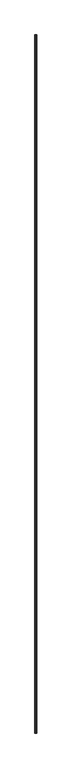
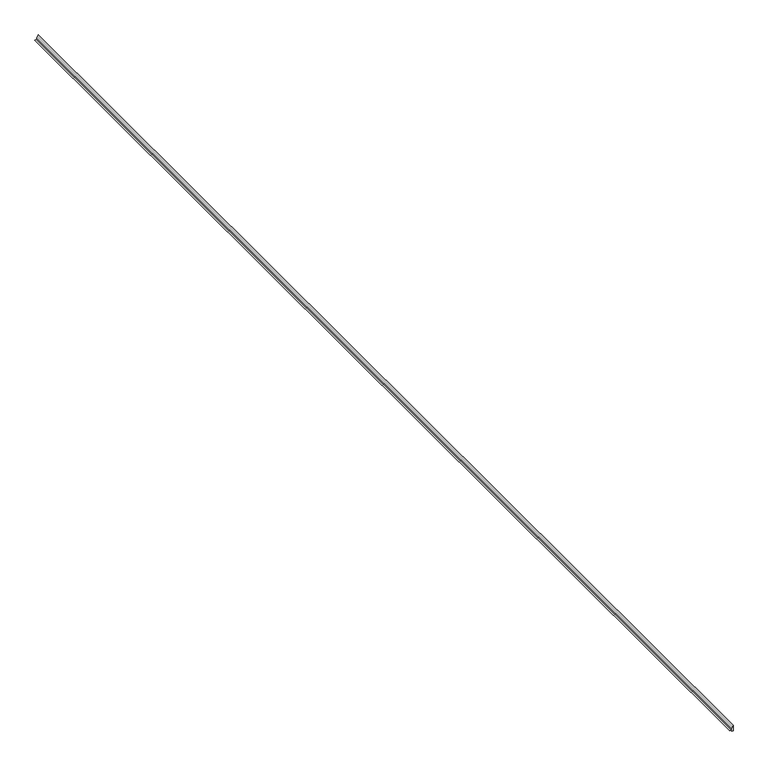
"""IFC4 building model written with IfcOpenShell, lengths in millimetres: proxy geometry, Generic Models 3:Generic Models 2:312240:Generic Models 2:312240 : Generic Models 3:Generic Models 2:312240:7 : Generic Models 3:Generic Models 2:312240:Generic Models 2:312240 : Generic Models 3:Generic Models 2:312240:300533."""

from ifc_helpers import new_model, si_unit, frame, origin, place, context, project, spatial, polyline, outline, extrude, source, transform, mapped, element, save


def generic_models_042a4f2a(model_context):
    return source(origin(), model_context, "Body", "SweptSolid", [
        extrude(outline(polyline([(0.0, 667585.4117239), (-2.5068284, 667585.4117239), (-2.5068284, 667587.6995663), (0.0, 667587.6995663), (9.4480138, 667587.6995663), (2.7766894, 667585.0041763), (1.5875, 667583.8149868), (0.0, 667581.0653562), (0.0, 667585.4117239)])), frame((0.0, -568496.2038841, 0.0), z_axis=(0.0, 1.0, 0.0), x_axis=(0.0, 0.0, 1.0)), (0.0, 0.0, 1.0), 2438.4),
    ])


if __name__ == "__main__":
    model = new_model("IFC4")
    model_context = context("Model", 3, world=origin())
    ifc_project = project(units=[si_unit("LENGTHUNIT", "METRE", prefix="MILLI")], contexts=[model_context])
    site = spatial("IfcSite", under=ifc_project)
    building = spatial("IfcBuilding", under=site)
    placement = place(None, origin())
    generic_models_shape = generic_models_042a4f2a(model_context)
    element("IfcBuildingElementProxy", 1, Name="Generic Models 3:Generic Models 2:312240:Generic Models 2:312240 : Generic Models 3:Generic Models 2:312240:7 : Generic Models 3:Generic Models 2:312240:Generic Models 2:312240 : Generic Models 3:Generic Models 2:312240:300533", ObjectType="Generic Models 3:Generic Models 2:312240:Generic Models 2:312240 : Generic Models 3:Generic Models 2:312240:7 : Generic Models 3:Generic Models 2:312240:Generic Models 2:312240 : Generic Models 3:Generic Models 2:312240:300533", at=placement, inside=building, context=model_context, shape_type="MappedRepresentation", body=[
        mapped(generic_models_shape, transform((0.0, 0.0, 0.0), x_axis=(1.0, 0.0, 0.0), y_axis=(0.0, 1.0, 0.0), z_axis=(0.0, 0.0, 1.0))),
    ])
    save(model, "model.ifc")

# Revit data of these elements
# Type "Generic Models 3:Generic Models 2:312240:Generic Models 2:312240 : Generic Models 3:Generic Models 2:312240:7 : Generic Models 3:Generic Models 2:312240:Generic Models 2:312240 : Generic Models 3:Generic Models 2:312240:300533"
#   NameOverride = "Generic Models 3:Generic Models 2:312240:Generic Models 2:312240 : Generic Models 3:Generic Models 2:312240:300533"
#   ObjectTypeOverride = "Generic Models 2:312240 : Generic Models 3:Generic Models 2:312240"
#   Reference = "Generic Models 2"
#   Tag = "300533"
# Element 1 (IfcBuildingElementProxy, "Generic Models 3:Generic Models 2:312240:Generic Models 2:312240 : Generic Models 3:Generic Models 2:312240:7 : Generic Models 3:Generic Models 2:312240:Generic Models 2:312240 : Generic Models 3:Generic Models 2:312240:300533")
#   Materials on its faces: "SEALANT & BACKER ROD, IF NECESSARY"
# Materials
#   "SEALANT & BACKER ROD, IF NECESSARY": class "Unassigned", colour RGB 120 120 120, transparency 0, Cost = 0
